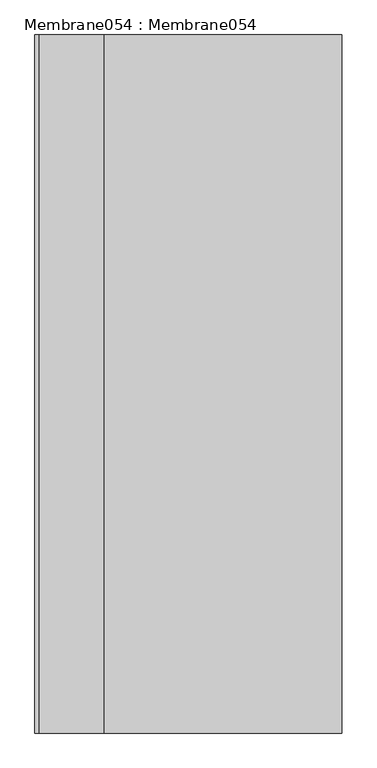
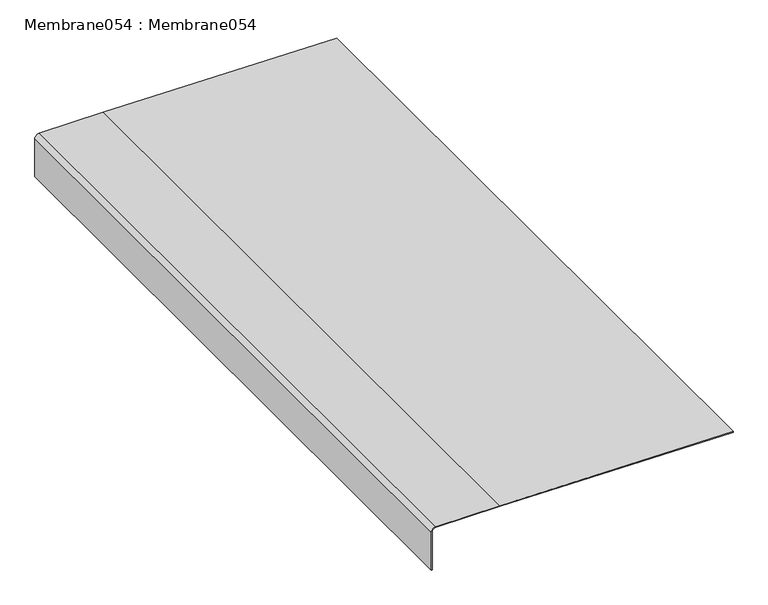
"""IFC4 building model written with IfcOpenShell, lengths in millimetres: proxy geometry, Membrane054 : Membrane054."""

from ifc_helpers import new_model, si_unit, point, frame, frame_2d, origin, place, context, project, spatial, polyline, circle_curve, trimmed, segment, composite_curve, outline, extrude, source, transform, mapped, element, save


def membrane054_membrane054_5bc26130(model_context):
    return source(origin(), model_context, "Body", "SweptSolid", [
        extrude(outline(composite_curve([segment(trimmed(circle_curve(frame_2d((40233.3001163, -2760.1593049)), 10.0), [point((40233.3001163, -2770.1593049))], [point((40243.3001163, -2760.1593049))], True, "CARTESIAN"), True, "CONTINUOUS"), segment(polyline([(40243.3001163, -2760.1593049), (40243.3001163, -2573.6408736), (40233.5063967, -1893.5405923), (40235.5061893, -1893.5117945), (40245.3001163, -2573.6264742), (40245.3001163, -2760.1593049)]), True, "CONTINUOUS"), segment(trimmed(circle_curve(frame_2d((40233.3001163, -2760.1593049)), 12.0), [point((40245.3001163, -2760.1593049))], [point((40233.3001163, -2772.1593049))], False, "CARTESIAN"), True, "CONTINUOUS"), segment(polyline([(40233.3001163, -2772.1593049), (40116.5801181, -2772.1593049), (40116.5801181, -2770.1593049), (40233.3001163, -2770.1593049)]), True, "CONTINUOUS")], self_intersect=False)), frame((0.0, -1052.8906574, 0.0), z_axis=(0.0, 1.0, 0.0), x_axis=(0.0, 0.0, 1.0)), (0.0, 0.0, 1.0), 2000.0),
    ])


if __name__ == "__main__":
    model = new_model("IFC4")
    model_context = context("Model", 3, world=origin())
    ifc_project = project(units=[si_unit("LENGTHUNIT", "METRE", prefix="MILLI")], contexts=[model_context])
    site = spatial("IfcSite", under=ifc_project)
    building = spatial("IfcBuilding", under=site)
    placement = place(None, origin())
    membrane054_membrane054_shape = membrane054_membrane054_5bc26130(model_context)
    element("IfcBuildingElementProxy", 1, Name="Membrane054 : Membrane054", ObjectType="Membrane054 : Membrane054", at=placement, inside=building, context=model_context, shape_type="MappedRepresentation", body=[
        mapped(membrane054_membrane054_shape, transform((0.0, 0.0, 0.0), x_axis=(1.0, 0.0, 0.0), y_axis=(0.0, 1.0, 0.0), z_axis=(0.0, 0.0, 1.0))),
    ])
    save(model, "model.ifc")

# Revit data of these elements
# Type "Membrane054 : Membrane054"
#   NameOverride = "Membrane054"
# Element 1 (IfcBuildingElementProxy, "Membrane054 : Membrane054")
#   Materials on its faces: "THREE PLY BUILT UP ROOF MEMBRANE"
# Materials
#   "THREE PLY BUILT UP ROOF MEMBRANE": class "Unassigned", colour RGB 63 63 63, transparency 0
